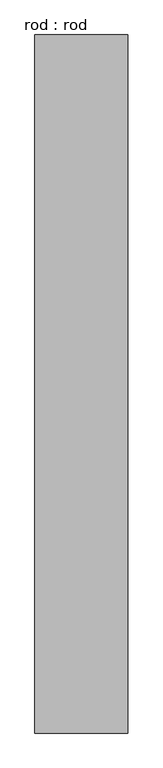
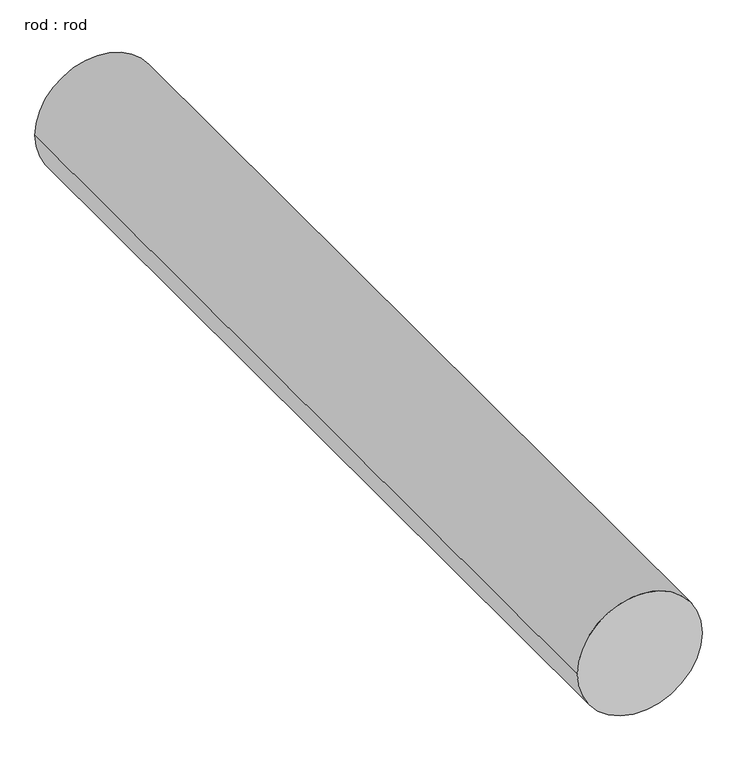
"""IFC4 building model written with IfcOpenShell, lengths in millimetres: proxy geometry, rod : rod."""

from ifc_helpers import new_model, si_unit, point, frame, frame_2d, origin, place, context, project, spatial, circle_curve, trimmed, segment, composite_curve, outline, extrude, source, transform, mapped, element, save


def rod_rod_562b52f6(model_context):
    return source(origin(), model_context, "Body", "SweptSolid", [
        extrude(outline(composite_curve([segment(trimmed(circle_curve(frame_2d((0.0108462, 0.0)), 200.0), [point((0.0108462, 200.0))], [point((0.0108462, -200.0))], False, "CARTESIAN"), True, "CONTINUOUS"), segment(trimmed(circle_curve(frame_2d((0.0108462, 0.0)), 200.0), [point((0.0108462, -200.0))], [point((0.0108462, 200.0))], False, "CARTESIAN"), True, "CONTINUOUS")], self_intersect=False)), frame((0.0, 2587.3714725, 0.0), z_axis=(0.0, 1.0, 0.0), x_axis=(0.0, 0.0, 1.0)), (0.0, 0.0, 1.0), 3010.7142857),
    ])


if __name__ == "__main__":
    model = new_model("IFC4")
    model_context = context("Model", 3, world=origin())
    ifc_project = project(units=[si_unit("LENGTHUNIT", "METRE", prefix="MILLI")], contexts=[model_context])
    site = spatial("IfcSite", under=ifc_project)
    building = spatial("IfcBuilding", under=site)
    placement = place(None, origin())
    rod_rod_shape = rod_rod_562b52f6(model_context)
    element("IfcBuildingElementProxy", 1, Name="rod : rod", ObjectType="rod : rod", at=placement, inside=building, context=model_context, shape_type="MappedRepresentation", body=[
        mapped(rod_rod_shape, transform((0.0, 0.0, 0.0), x_axis=(1.0, 0.0, 0.0), y_axis=(0.0, 1.0, 0.0), z_axis=(0.0, 0.0, 1.0))),
    ])
    save(model, "model.ifc")

# Revit data of these elements
# Type "rod : rod"
#   Default Elevation = 0
